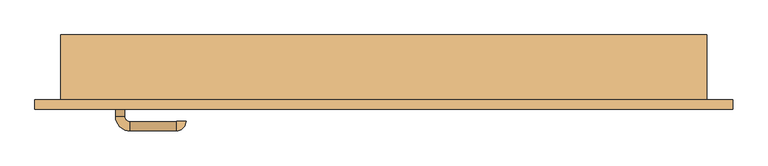
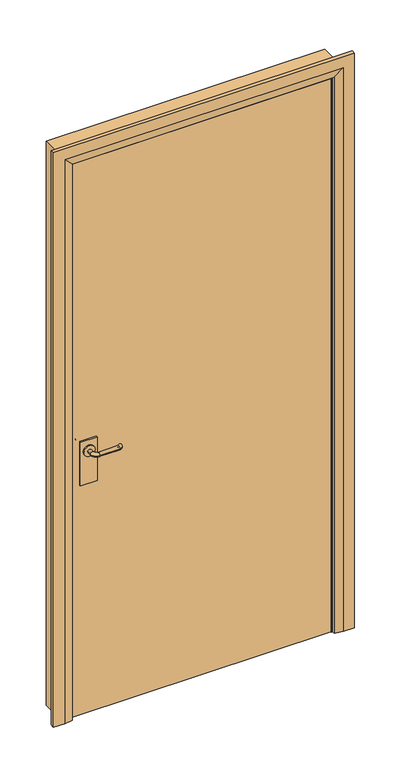
"""IFC4 building model written with IfcOpenShell, lengths in millimetres: door geometry, Porta Simples de Abrir : 90x210cm - Aduela de Madeira."""

from ifc_helpers import new_model, si_unit, point, frame, frame_2d, origin, place, context, project, spatial, polyline, circle_curve, ellipse_curve, trimmed, segment, composite_curve, outline, extrude, faceted_brep, source, transform, mapped, element, save
from ifc_brep_helpers import plane_surface, cylinder_surface, revolved_surface, advanced_brep


def door_267b7e8a(model_context):
    return source(origin(), model_context, "Body", "SolidModel", [
        extrude(outline(composite_curve([segment(trimmed(circle_curve(frame_2d((1050.0, -408.0)), 20.0), [point((1050.0, -428.0))], [point((1050.0, -388.0))], False, "CARTESIAN"), True, "CONTINUOUS"), segment(trimmed(circle_curve(frame_2d((1050.0, -408.0)), 20.0), [point((1050.0, -388.0))], [point((1050.0, -428.0))], False, "CARTESIAN"), True, "CONTINUOUS")], self_intersect=False)), frame((0.0, -44.6, 0.0), z_axis=(0.0, 1.0, 0.0), x_axis=(0.0, 0.0, 1.0)), (0.0, 0.0, 1.0), 4.5929895),
        advanced_brep(
        [(-401.0, -40.0070105, 1050.0), (-415.0, -40.0070105, 1050.0), (-401.0, -24.6, 1050.0), (-415.0, -24.6, 1050.0), (-393.0, -2.6, 1050.0), (-393.0, -16.6, 1050.0), (-321.0, -16.6, 1050.0), (-321.0, -2.6, 1050.0), (-320.0, -17.6, 1050.0), (-306.0, -17.6, 1050.0)],
        [
            (0, 1, circle_curve(frame((-408.0, -40.0070105, 1050.0), z_axis=(0.0, -1.0, 0.0), x_axis=(-1.0, 0.0, 0.0)), 7.0)),
            (1, 0, circle_curve(frame((-408.0, -40.0070105, 1050.0), z_axis=(0.0, -1.0, 0.0), x_axis=(-1.0, 0.0, 0.0)), 7.0)),
            (0, 2),
            (2, 3, circle_curve(frame((-408.0, -24.6, 1050.0), z_axis=(0.0, -1.0, 0.0), x_axis=(-1.0, 0.0, 0.0)), 7.0)),
            (3, 1),
            (3, 2, circle_curve(frame((-408.0, -24.6, 1050.0), z_axis=(0.0, -1.0, 0.0), x_axis=(-1.0, 0.0, 0.0)), 7.0)),
            (4, 3, circle_curve(frame((-393.0, -24.6, 1050.0), z_axis=(0.0, 0.0, 1.0), x_axis=(-1.0, 0.0, 0.0)), 22.0)),
            (2, 5, circle_curve(frame((-393.0, -24.6, 1050.0), z_axis=(0.0, 0.0, -1.0), x_axis=(-1.0, 0.0, 0.0)), 8.0)),
            (5, 4, circle_curve(frame((-393.0, -9.6, 1050.0), z_axis=(-1.0, 0.0, 0.0), x_axis=(0.0, 1.0, 0.0)), 7.0)),
            (4, 5, circle_curve(frame((-393.0, -9.6, 1050.0), z_axis=(-1.0, 0.0, 0.0), x_axis=(0.0, 1.0, 0.0)), 7.0)),
            (5, 6),
            (6, 7, circle_curve(frame((-321.0, -9.6, 1050.0), z_axis=(-1.0, 0.0, 0.0), x_axis=(0.0, 1.0, 0.0)), 7.0)),
            (7, 4),
            (7, 6, circle_curve(frame((-321.0, -9.6, 1050.0), z_axis=(-1.0, 0.0, 0.0), x_axis=(0.0, 1.0, 0.0)), 7.0)),
            (8, 9, circle_curve(frame((-313.0, -17.6, 1050.0), z_axis=(0.0, -1.0, 0.0), x_axis=(1.0, 0.0, 0.0)), 7.0)),
            (9, 8, circle_curve(frame((-313.0, -17.6, 1050.0), z_axis=(0.0, -1.0, 0.0), x_axis=(1.0, 0.0, 0.0)), 7.0)),
            (9, 7, circle_curve(frame((-321.0, -17.6, 1050.0), z_axis=(0.0, 0.0, 1.0), x_axis=(0.0, 1.0, 0.0)), 15.0)),
            (6, 8, circle_curve(frame((-321.0, -17.6, 1050.0), z_axis=(0.0, 0.0, -1.0), x_axis=(0.0, 1.0, 0.0)), 1.0)),
        ],
        [
            plane_surface(frame((-408.0, -40.0070105, 1050.0), z_axis=(0.0, -1.0, 0.0), x_axis=(0.0, 0.0, 1.0))),
            cylinder_surface(frame((-408.0, -40.0070105, 1050.0), z_axis=(0.0, -1.0, 0.0), x_axis=(-1.0, 0.0, 0.0)), 7.0),
            revolved_surface(trimmed(ellipse_curve(frame((-408.0, -24.6, 1050.0), z_axis=(0.0, -1.0, 0.0), x_axis=(-1.0, 0.0, 0.0)), 7.0, 7.0), [point((-401.0, -24.6, 1050.0))], [point((-415.0, -24.6, 1050.0))], True, "CARTESIAN"), (-393.0, -24.6, 1050.0), (0.0, 0.0, -1.0)),
            revolved_surface(trimmed(ellipse_curve(frame((-408.0, -24.6, 1050.0), z_axis=(0.0, -1.0, 0.0), x_axis=(-1.0, 0.0, 0.0)), 7.0, 7.0), [point((-415.0, -24.6, 1050.0))], [point((-401.0, -24.6, 1050.0))], True, "CARTESIAN"), (-393.0, -24.6, 1050.0), (0.0, 0.0, -1.0)),
            cylinder_surface(frame((-393.0, -9.6, 1050.0), z_axis=(-1.0, 0.0, 0.0), x_axis=(0.0, 1.0, 0.0)), 7.0),
            plane_surface(frame((-313.0, -17.6, 1050.0), z_axis=(0.0, -1.0, 0.0), x_axis=(0.0, 0.0, 1.0))),
            revolved_surface(trimmed(ellipse_curve(frame((-321.0, -9.6, 1050.0), z_axis=(-1.0, 0.0, 0.0), x_axis=(0.0, 1.0, 0.0)), 7.0, 7.0), [point((-321.0, -16.6, 1050.0))], [point((-321.0, -2.6, 1050.0))], True, "CARTESIAN"), (-321.0, -17.6, 1050.0), (0.0, 0.0, -1.0)),
            revolved_surface(trimmed(ellipse_curve(frame((-321.0, -9.6, 1050.0), z_axis=(-1.0, 0.0, 0.0), x_axis=(0.0, 1.0, 0.0)), 7.0, 7.0), [point((-321.0, -2.6, 1050.0))], [point((-321.0, -16.6, 1050.0))], True, "CARTESIAN"), (-321.0, -17.6, 1050.0), (0.0, 0.0, -1.0)),
        ],
        [
            (0, [[1, 2]]),
            (1, [[-1, 3, 4, 5]]),
            (1, [[-2, -5, 6, -3]]),
            (2, [[7, -4, 8, 9]]),
            (3, [[-8, -6, -7, 10]]),
            (4, [[-9, 11, 12, 13]]),
            (4, [[-10, -13, 14, -11]]),
            (5, [[15, 16]]),
            (6, [[17, -12, 18, -16]]),
            (7, [[-18, -14, -17, -15]]),
        ],
    ),
        extrude(outline(polyline([(-378.0, -50.6), (-438.0, -50.6), (-438.0, -44.6), (-378.0, -44.6), (-378.0, -50.6)])), frame((0.0, 0.0, 925.0), z_axis=(0.0, 0.0, 1.0), x_axis=(1.0, 0.0, 0.0)), (0.0, 0.0, 1.0), 165.0),
        extrude(outline(composite_curve([segment(trimmed(circle_curve(frame_2d((1050.0, -408.0)), 20.0), [point((1050.0, -428.0))], [point((1050.0, -388.0))], False, "CARTESIAN"), True, "CONTINUOUS"), segment(trimmed(circle_curve(frame_2d((1050.0, -408.0)), 20.0), [point((1050.0, -388.0))], [point((1050.0, -428.0))], False, "CARTESIAN"), True, "CONTINUOUS")], self_intersect=False)), frame((0.0, -96.1929895, 0.0), z_axis=(0.0, 1.0, 0.0), x_axis=(0.0, 0.0, 1.0)), (0.0, 0.0, 1.0), 4.5929895),
        advanced_brep(
        [(-401.0, -96.1929895, 1050.0), (-415.0, -96.1929895, 1050.0), (-415.0, -111.6, 1050.0), (-401.0, -111.6, 1050.0), (-393.0, -133.6, 1050.0), (-393.0, -119.6, 1050.0), (-321.0, -133.6, 1050.0), (-321.0, -119.6, 1050.0), (-320.0, -118.6, 1050.0), (-306.0, -118.6, 1050.0)],
        [
            (0, 1, circle_curve(frame((-408.0, -96.1929895, 1050.0), z_axis=(0.0, 1.0, 0.0), x_axis=(-1.0, 0.0, 0.0)), 7.0)),
            (1, 0, circle_curve(frame((-408.0, -96.1929895, 1050.0), z_axis=(0.0, 1.0, 0.0), x_axis=(-1.0, 0.0, 0.0)), 7.0)),
            (1, 2),
            (2, 3, circle_curve(frame((-408.0, -111.6, 1050.0), z_axis=(0.0, 1.0, 0.0), x_axis=(-1.0, 0.0, 0.0)), 7.0)),
            (3, 0),
            (3, 2, circle_curve(frame((-408.0, -111.6, 1050.0), z_axis=(0.0, 1.0, 0.0), x_axis=(-1.0, 0.0, 0.0)), 7.0)),
            (4, 5, circle_curve(frame((-393.0, -126.6, 1050.0), z_axis=(-1.0, 0.0, 0.0), x_axis=(0.0, -1.0, 0.0)), 7.0)),
            (5, 3, circle_curve(frame((-393.0, -111.6, 1050.0), z_axis=(0.0, 0.0, -1.0), x_axis=(-1.0, 0.0, 0.0)), 8.0)),
            (2, 4, circle_curve(frame((-393.0, -111.6, 1050.0), z_axis=(0.0, 0.0, 1.0), x_axis=(-1.0, 0.0, 0.0)), 22.0)),
            (5, 4, circle_curve(frame((-393.0, -126.6, 1050.0), z_axis=(-1.0, 0.0, 0.0), x_axis=(0.0, -1.0, 0.0)), 7.0)),
            (4, 6),
            (6, 7, circle_curve(frame((-321.0, -126.6, 1050.0), z_axis=(-1.0, 0.0, 0.0), x_axis=(0.0, -1.0, 0.0)), 7.0)),
            (7, 5),
            (7, 6, circle_curve(frame((-321.0, -126.6, 1050.0), z_axis=(-1.0, 0.0, 0.0), x_axis=(0.0, -1.0, 0.0)), 7.0)),
            (8, 9, circle_curve(frame((-313.0, -118.6, 1050.0), z_axis=(0.0, 1.0, 0.0), x_axis=(1.0, 0.0, 0.0)), 7.0)),
            (9, 8, circle_curve(frame((-313.0, -118.6, 1050.0), z_axis=(0.0, 1.0, 0.0), x_axis=(1.0, 0.0, 0.0)), 7.0)),
            (8, 7, circle_curve(frame((-321.0, -118.6, 1050.0), z_axis=(0.0, 0.0, -1.0), x_axis=(0.0, -1.0, 0.0)), 1.0)),
            (6, 9, circle_curve(frame((-321.0, -118.6, 1050.0), z_axis=(0.0, 0.0, 1.0), x_axis=(0.0, -1.0, 0.0)), 15.0)),
        ],
        [
            plane_surface(frame((-408.0, -96.1929895, 1050.0), z_axis=(0.0, 1.0, 0.0), x_axis=(0.0, 0.0, 1.0))),
            cylinder_surface(frame((-408.0, -96.1929895, 1050.0), z_axis=(0.0, 1.0, 0.0), x_axis=(-1.0, 0.0, 0.0)), 7.0),
            revolved_surface(trimmed(ellipse_curve(frame((-408.0, -111.6, 1050.0), z_axis=(0.0, -1.0, 0.0), x_axis=(-1.0, 0.0, 0.0)), 7.0, 7.0), [point((-401.0, -111.6, 1050.0))], [point((-415.0, -111.6, 1050.0))], True, "CARTESIAN"), (-393.0, -111.6, 1050.0), (0.0, 0.0, -1.0)),
            revolved_surface(trimmed(ellipse_curve(frame((-408.0, -111.6, 1050.0), z_axis=(0.0, -1.0, 0.0), x_axis=(-1.0, 0.0, 0.0)), 7.0, 7.0), [point((-415.0, -111.6, 1050.0))], [point((-401.0, -111.6, 1050.0))], True, "CARTESIAN"), (-393.0, -111.6, 1050.0), (0.0, 0.0, -1.0)),
            cylinder_surface(frame((-393.0, -126.6, 1050.0), z_axis=(-1.0, 0.0, 0.0), x_axis=(0.0, -1.0, 0.0)), 7.0),
            plane_surface(frame((-313.0, -118.6, 1050.0), z_axis=(0.0, 1.0, 0.0), x_axis=(0.0, 0.0, 1.0))),
            revolved_surface(trimmed(ellipse_curve(frame((-321.0, -126.6, 1050.0), z_axis=(1.0, 0.0, 0.0), x_axis=(0.0, -1.0, 0.0)), 7.0, 7.0), [point((-321.0, -119.6, 1050.0))], [point((-321.0, -133.6, 1050.0))], True, "CARTESIAN"), (-321.0, -118.6, 1050.0), (0.0, 0.0, -1.0)),
            revolved_surface(trimmed(ellipse_curve(frame((-321.0, -126.6, 1050.0), z_axis=(1.0, 0.0, 0.0), x_axis=(0.0, -1.0, 0.0)), 7.0, 7.0), [point((-321.0, -133.6, 1050.0))], [point((-321.0, -119.6, 1050.0))], True, "CARTESIAN"), (-321.0, -118.6, 1050.0), (0.0, 0.0, -1.0)),
        ],
        [
            (0, [[1, 2]]),
            (1, [[3, 4, 5, -2]]),
            (1, [[-5, 6, -3, -1]]),
            (2, [[7, 8, -4, 9]]),
            (3, [[10, -9, -6, -8]]),
            (4, [[11, 12, 13, -7]]),
            (4, [[-13, 14, -11, -10]]),
            (5, [[15, 16]]),
            (6, [[-15, 17, -12, 18]]),
            (7, [[-16, -18, -14, -17]]),
        ],
    ),
        extrude(outline(polyline([(-378.0, -85.6), (-378.0, -91.6), (-438.0, -91.6), (-438.0, -85.6), (-378.0, -85.6)])), frame((0.0, 0.0, 925.0), z_axis=(0.0, 0.0, 1.0), x_axis=(1.0, 0.0, 0.0)), (0.0, 0.0, 1.0), 165.0),
        extrude(outline(polyline([(463.0, -50.6), (463.0, -85.6), (-463.0, -85.6), (-463.0, -50.6), (463.0, -50.6)])), frame((0.0, 0.0, 53.0), z_axis=(0.0, 0.0, 1.0), x_axis=(1.0, 0.0, 0.0)), (0.0, 0.0, 1.0), 2099.0),
        faceted_brep([(540.0, -85.6, 50.0), (540.0, -100.6, 50.0), (500.0, -100.6, 50.0), (470.0, -95.6, 50.0), (470.0, -85.6, 50.0), (470.0, -85.6, 2160.0), (-470.0, -85.6, 2160.0), (-470.0, -85.6, 50.0), (-540.0, -85.6, 50.0), (-540.0, -85.6, 2230.0), (540.0, -85.6, 2230.0), (470.0, -95.6, 2160.0), (500.0, -100.6, 2190.0), (540.0, -100.6, 2230.0), (-540.0, -100.6, 2230.0), (-540.0, -100.6, 50.0), (-500.0, -100.6, 50.0), (-500.0, -100.6, 2190.0), (-470.0, -95.6, 50.0), (-470.0, -95.6, 2160.0)], [[[0, 1, 2, 3, 4]], [[4, 5, 6, 7, 8, 9, 10, 0]], [[3, 11, 5, 4]], [[2, 12, 11, 3]], [[1, 13, 14, 15, 16, 17, 12, 2]], [[0, 10, 13, 1]], [[9, 8, 15, 14]], [[8, 7, 18, 16, 15]], [[19, 18, 7, 6]], [[17, 16, 18, 19]], [[11, 19, 6, 5]], [[10, 9, 14, 13]], [[12, 17, 19, 11]]]),
        faceted_brep([(-465.0, -85.6, 50.0), (-500.0, -85.6, 50.0), (-500.0, 14.4, 50.0), (-455.0, 14.4, 50.0), (-455.0, -48.6, 50.0), (-465.0, -48.6, 50.0), (-465.0, -48.6, 2155.0), (-465.0, -85.6, 2155.0), (-455.0, -48.6, 2145.0), (455.0, -48.6, 2145.0), (455.0, -48.6, 50.0), (465.0, -48.6, 50.0), (465.0, -48.6, 2155.0), (-455.0, 14.4, 2145.0), (-500.0, 14.4, 2190.0), (500.0, 14.4, 2190.0), (500.0, 14.4, 50.0), (455.0, 14.4, 50.0), (455.0, 14.4, 2145.0), (-500.0, -85.6, 2190.0), (465.0, -85.6, 2155.0), (465.0, -85.6, 50.0), (500.0, -85.6, 50.0), (500.0, -85.6, 2190.0)], [[[0, 1, 2, 3, 4, 5]], [[5, 6, 7, 0]], [[4, 8, 9, 10, 11, 12, 6, 5]], [[3, 13, 8, 4]], [[2, 14, 15, 16, 17, 18, 13, 3]], [[1, 19, 14, 2]], [[0, 7, 20, 21, 22, 23, 19, 1]], [[12, 11, 21, 20]], [[21, 11, 10, 17, 16, 22]], [[18, 17, 10, 9]], [[23, 22, 16, 15]], [[6, 12, 20, 7]], [[13, 18, 9, 8]], [[19, 23, 15, 14]]]),
    ])


if __name__ == "__main__":
    model = new_model("IFC4")
    model_context = context("Model", 3, world=origin())
    ifc_project = project(units=[si_unit("LENGTHUNIT", "METRE", prefix="MILLI")], contexts=[model_context])
    site = spatial("IfcSite", under=ifc_project)
    building = spatial("IfcBuilding", under=site)
    placement = place(None, origin())
    door_shape = door_267b7e8a(model_context)
    element("IfcDoor", 1, ObjectType="Porta Simples de Abrir : 90x210cm - Aduela de Madeira", at=placement, inside=building, context=model_context, shape_type="MappedRepresentation", body=[
        mapped(door_shape, transform((0.0, 0.0, 0.0), x_axis=(1.0, 0.0, 0.0), y_axis=(0.0, 1.0, 0.0), z_axis=(0.0, 0.0, 1.0))),
    ])
    save(model, "model.ifc")

# Revit data of these elements
# Type "Porta Simples de Abrir : 90x210cm - Aduela de Madeira"
#   Type Mark = ""
#   SINAPI = ""
#   Construction Type = "300"
#   Maçaneta [instance default] = ""
#   Fechadura [instance default] = ""
#   Vão Luz (somente para informação) = 89.00 cm
#   Tolerância Folha Vertical = 0.30 cm
#   Módulo Básico M = 10.00 cm
#   Largura de Coordenação Modular Largura CM = 100.00 cm
#   Rough Width = 100.00 cm
#   Deslocamento da Horizontal da Folha = 0.00 cm
#   Altura de Coordenação Modular Largura CM = 220.00 cm
#   Rough Height = 220.00 cm
#   Altura Nominal = 209.50 cm
#   Ajuste de Coordenação Topo AC Topo = 1.00 cm
#   Ajuste de Coordenação Base AC Base = 5.00 cm
#   Ajuste de Coordenação AC = 1.00 cm
#   Tolerância Folha Horizontal = 0.20 cm
#   Largura Folha (somente para informação) = 90.60 cm
#   Espessura Folha = 3.50 cm
#   Maçaneta - Distância da Folha = 5.50 cm
#   Maçaneta - Altura = 100.00 cm
#   Largura Nominal (Largura Mn) = 93.00 cm
#   Distância do Nível = 0.30 cm
#   Aduela Interna Espessura = 3.50 cm
#   Aduela Externa Espessura = 4.50 cm
#   Altura Folha (somente para informação) = 208.00 cm
#   Height = 214.00 cm
#   Width = 98.00 cm
#   Número de Módulos Básicos nM Largura = 10
#   Número de Módulos Básicos nM Altura = 22
#   Marco Metálico = no
#   Aduela de Madeira = yes
#   Aduela Metálica de Canto = no
#   Guarnição Reta = no
#   Guarnição Chanfrada = no
#   Batente - Material [instance default] = none
#   Painel - Material [instance default] = none
#   Model = ""
#   Function = (empty or 0)
#   Description = (empty or 0)
#   Wall Closure = (empty or 0)
#   Assembly Code = ""
# Element 1 (IfcDoor, "Porta Simples de Abrir : 90x210cm - Aduela de Madeira")
#   Materials on its faces: "Porta - Maçaneta"
# Materials
#   "Porta - Maçaneta": class "Metal", colour RGB 189 187 185, transparency 0, Cost = 0
